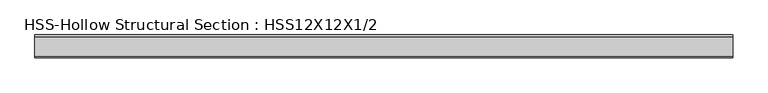
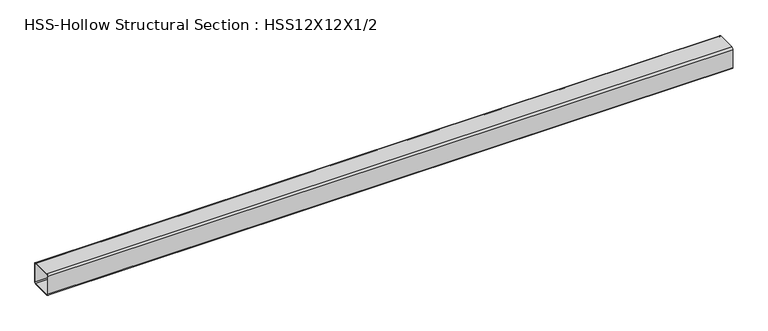
"""IFC4 building model written with IfcOpenShell, lengths in millimetres: beam geometry, HSS-Hollow Structural Section : HSS12X12X1/2."""

import ifcopenshell
import ifcopenshell.guid

model = None  # the IFC model being written
_history = None  # IfcOwnerHistory: only IFC2X3 demands one
_inside = {}  # id of a spatial element -> (the spatial element, [elements in it])
_under = {}  # id of a project, library or spatial element -> (it, [spatial elements below it])
_declared = {}  # id of a project -> (the project, [libraries it declares])
_typed = {}  # id of a type object -> (the type object, [elements of that type])
_made_of = {}  # id of a material, layer set ... -> (it, [elements and type objects made of it])


def new_model(schema):
    """Start an empty IFC model of exactly this schema.

    Asked for "IFC4X3", IfcOpenShell would pick the latest addendum, in which some entities
    have other attributes; the version numbers below select the first issue.
    IFC2X3 requires an IfcOwnerHistory on every rooted entity: one is made here for all.
    """
    global model, _history
    if schema == "IFC4X3":
        model = ifcopenshell.file(schema_version=(4, 3, 0, 0))
    else:
        model = ifcopenshell.file(schema=schema)
    _inside.clear()
    _under.clear()
    _declared.clear()
    _typed.clear()
    _made_of.clear()
    _history = None
    if model.schema == "IFC2X3":
        org = make("IfcOrganization", Name="unknown")
        user = make(
            "IfcPersonAndOrganization",
            ThePerson=make("IfcPerson", FamilyName="unknown"),
            TheOrganization=org,
        )
        app = make(
            "IfcApplication",
            ApplicationDeveloper=org,
            Version="unknown",
            ApplicationFullName="unknown",
            ApplicationIdentifier="unknown",
        )
        _history = make(
            "IfcOwnerHistory",
            OwningUser=user,
            OwningApplication=app,
            ChangeAction="ADDED",
            CreationDate=0,
        )
    return model


def make(cls, **values):
    """One entity of the class cls with the attributes given. An attribute that is None is left unset."""
    return model.create_entity(
        cls, **{name: value for name, value in values.items() if value is not None}
    )


def rooted(cls, **values):
    """An entity with a GlobalId (a new one), such as an element, a storey or a relation."""
    return make(cls, GlobalId=ifcopenshell.guid.new(), OwnerHistory=_history, **values)


def si_unit(unit_type, name, prefix=None):
    """IfcSIUnit, for example si_unit("LENGTHUNIT", "METRE", prefix="MILLI")."""
    return make("IfcSIUnit", UnitType=unit_type, Prefix=prefix, Name=name)


def assignment(units):
    """IfcUnitAssignment: the units of a project."""
    return None if units is None else make("IfcUnitAssignment", Units=units)


def point(xyz):
    """IfcCartesianPoint."""
    return None if xyz is None else make("IfcCartesianPoint", Coordinates=xyz)


def direction(xyz):
    """IfcDirection."""
    return None if xyz is None else make("IfcDirection", DirectionRatios=xyz)


def frame(location, z_axis=None, x_axis=None):
    """IfcAxis2Placement3D, a coordinate frame: its origin and axes. An axis left out is left unset."""
    return make(
        "IfcAxis2Placement3D",
        Location=point(location),
        Axis=direction(z_axis),
        RefDirection=direction(x_axis),
    )


def frame_2d(location, x_axis=None):
    """IfcAxis2Placement2D, a coordinate frame in the plane: its origin and x axis."""
    return make(
        "IfcAxis2Placement2D", Location=point(location), RefDirection=direction(x_axis)
    )


def origin():
    """The frame at (0, 0, 0) with its axes left unset."""
    return frame((0.0, 0.0, 0.0))


def place(relative_to, where):
    """IfcLocalPlacement: puts the frame where relative to a parent placement (None: the world)."""
    return make(
        "IfcLocalPlacement", PlacementRelTo=relative_to, RelativePlacement=where
    )


def context(
    kind, dimensions, precision=None, world=None, true_north=None, identifier=None
):
    """IfcGeometricRepresentationContext, for example the 3D "Model" context."""
    return make(
        "IfcGeometricRepresentationContext",
        ContextIdentifier=identifier,
        ContextType=kind,
        CoordinateSpaceDimension=dimensions,
        Precision=precision,
        WorldCoordinateSystem=world,
        TrueNorth=true_north,
    )


def project(units=None, contexts=None):
    """IfcProject with its units and contexts."""
    return rooted(
        "IfcProject",
        Name="project",
        RepresentationContexts=contexts,
        UnitsInContext=assignment(units),
    )


def spatial(cls, under=None, at=None, **own):
    """A site, building, storey or space (cls), placed at a placement, below another one or the project."""
    s = rooted(cls, ObjectPlacement=at, **own)
    if under is not None:
        _under.setdefault(under.id(), (under, []))[1].append(s)
    return s


def polyline(points):
    """IfcPolyline through the points."""
    return make("IfcPolyline", Points=[point(p) for p in points])


def circle_curve(where, radius):
    """IfcCircle in the frame where."""
    return make("IfcCircle", Position=where, Radius=radius)


def trimmed(basis, trim1, trim2, sense, master):
    """IfcTrimmedCurve: the piece of a basis curve between two trims."""
    return make(
        "IfcTrimmedCurve",
        BasisCurve=basis,
        Trim1=trim1,
        Trim2=trim2,
        SenseAgreement=sense,
        MasterRepresentation=master,
    )


def segment(curve, same_sense, transition):
    """IfcCompositeCurveSegment."""
    return make(
        "IfcCompositeCurveSegment",
        Transition=transition,
        SameSense=same_sense,
        ParentCurve=curve,
    )


def composite_curve(segments, self_intersect=None):
    """IfcCompositeCurve: segments joined end to end."""
    return make("IfcCompositeCurve", Segments=segments, SelfIntersect=self_intersect)


def outline(outer, holes=None, kind="AREA"):
    """IfcArbitraryClosedProfileDef: a profile drawn as a closed curve; with holes, ...WithVoids."""
    if holes is None:
        return make("IfcArbitraryClosedProfileDef", ProfileType=kind, OuterCurve=outer)
    return make(
        "IfcArbitraryProfileDefWithVoids",
        ProfileType=kind,
        OuterCurve=outer,
        InnerCurves=holes,
    )


def extrude(swept, where, along, depth):
    """IfcExtrudedAreaSolid: the profile swept, set in the frame where, extruded along a direction by depth."""
    return make(
        "IfcExtrudedAreaSolid",
        SweptArea=swept,
        Position=where,
        ExtrudedDirection=direction(along),
        Depth=depth,
    )


def shape(context_of_items, identifier, shape_type, items):
    """IfcShapeRepresentation: the items that make up one representation, for example the "Body"."""
    return make(
        "IfcShapeRepresentation",
        ContextOfItems=context_of_items,
        RepresentationIdentifier=identifier,
        RepresentationType=shape_type,
        Items=items,
    )


def source(mapping_origin, context_of_items, identifier, shape_type, items):
    """IfcRepresentationMap: a shape defined once, which mapped items show again and again."""
    return make(
        "IfcRepresentationMap",
        MappingOrigin=mapping_origin,
        MappedRepresentation=shape(context_of_items, identifier, shape_type, items),
    )


def transform(
    local_origin,
    x_axis=None,
    y_axis=None,
    z_axis=None,
    scale=None,
    scale2=None,
    scale3=None,
    uniform=True,
):
    """IfcCartesianTransformationOperator3D, or its non-uniform kind. x_axis, y_axis, z_axis: its Axis1, 2, 3."""
    if uniform:
        return make(
            "IfcCartesianTransformationOperator3D",
            Axis1=direction(x_axis),
            Axis2=direction(y_axis),
            LocalOrigin=point(local_origin),
            Scale=scale,
            Axis3=direction(z_axis),
        )
    return make(
        "IfcCartesianTransformationOperator3DnonUniform",
        Axis1=direction(x_axis),
        Axis2=direction(y_axis),
        LocalOrigin=point(local_origin),
        Scale=scale,
        Axis3=direction(z_axis),
        Scale2=scale2,
        Scale3=scale3,
    )


def mapped(mapping_source, mapping_target):
    """IfcMappedItem: shows the shape of a source again, moved by a transform."""
    return make(
        "IfcMappedItem", MappingSource=mapping_source, MappingTarget=mapping_target
    )


def made_of(thing, what):
    """Note that an element or type object is made of a material, layer set ...; save() writes the relation."""
    if what is not None:
        _made_of.setdefault(what.id(), (what, []))[1].append(thing)
    return thing


def element(
    cls,
    number,
    at=None,
    inside=None,
    cuts=None,
    type_object=None,
    material=None,
    context=None,
    identifier="Body",
    shape_type=None,
    held_by="IfcProductDefinitionShape",
    body=None,
    shapes=None,
    **own,
):
    """One element of the class cls, such as IfcWall. Its Tag is "e" and its number.

    at: its placement. inside: the storey or other place that contains it. cuts: it is an
    opening in that element (IfcRelVoidsElement). A single representation is given by context,
    identifier, shape_type and body (its items); several are given by shapes. held_by: the class
    of the entity that holds the representations. save() writes the other relations.
    """
    e = rooted(cls, Tag="e%d" % number, ObjectPlacement=at, **own)
    if body is not None:
        shapes = [shape(context, identifier, shape_type, body)]
    if shapes is not None:
        e.Representation = make(held_by, Representations=shapes)
    if inside is not None:
        _inside.setdefault(inside.id(), (inside, []))[1].append(e)
    if cuts is not None:
        rooted(
            "IfcRelVoidsElement", RelatingBuildingElement=cuts, RelatedOpeningElement=e
        )
    if type_object is not None:
        _typed.setdefault(type_object.id(), (type_object, []))[1].append(e)
    return made_of(e, material)


def aggregate(whole, parts):
    """IfcRelAggregates: a whole, such as a stair, and the parts it consists of."""
    return rooted("IfcRelAggregates", RelatingObject=whole, RelatedObjects=parts)


def save(model, path):
    """Write the relations noted so far, then the file.

    IfcRelAggregates (storeys below a building ...), IfcRelContainedInSpatialStructure (elements
    in a storey), IfcRelDefinesByType, IfcRelAssociatesMaterial and IfcRelDeclares: one each for
    every whole, place, type object, material and project.
    """
    for whole, parts in _under.values():
        aggregate(whole, parts)
    for where, things in _inside.values():
        rooted(
            "IfcRelContainedInSpatialStructure",
            RelatedElements=things,
            RelatingStructure=where,
        )
    for kind, things in _typed.values():
        rooted("IfcRelDefinesByType", RelatedObjects=things, RelatingType=kind)
    for what, things in _made_of.values():
        rooted("IfcRelAssociatesMaterial", RelatedObjects=things, RelatingMaterial=what)
    for by, libraries in _declared.values():
        rooted("IfcRelDeclares", RelatingContext=by, RelatedDefinitions=libraries)
    model.write(path)


def hss_hollow_structural_section_hss12x12x1_2_15489e63(model_context):
    return source(origin(), model_context, "Body", "SweptSolid", [
        extrude(outline(composite_curve([segment(polyline([(152.4, 128.778), (152.4, -128.778)]), True, "CONTINUOUS"), segment(trimmed(circle_curve(frame_2d((128.778, -128.778)), 23.622), [point((152.4, -128.778))], [point((128.778, -152.4))], False, "CARTESIAN"), True, "CONTINUOUS"), segment(polyline([(128.778, -152.4), (-128.778, -152.4)]), True, "CONTINUOUS"), segment(trimmed(circle_curve(frame_2d((-128.778, -128.778)), 23.622), [point((-128.778, -152.4))], [point((-152.4, -128.778))], False, "CARTESIAN"), True, "CONTINUOUS"), segment(polyline([(-152.4, -128.778), (-152.4, 128.778)]), True, "CONTINUOUS"), segment(trimmed(circle_curve(frame_2d((-128.778, 128.778)), 23.622), [point((-152.4, 128.778))], [point((-128.778, 152.4))], False, "CARTESIAN"), True, "CONTINUOUS"), segment(polyline([(-128.778, 152.4), (128.778, 152.4)]), True, "CONTINUOUS"), segment(trimmed(circle_curve(frame_2d((128.778, 128.778)), 23.622), [point((128.778, 152.4))], [point((152.4, 128.778))], False, "CARTESIAN"), True, "CONTINUOUS")], self_intersect=False), holes=[composite_curve([segment(trimmed(circle_curve(frame_2d((-128.778, 128.778)), 11.811), [point((-128.778, 140.589))], [point((-140.589, 128.778))], True, "CARTESIAN"), True, "CONTINUOUS"), segment(polyline([(-140.589, 128.778), (-140.589, -128.778)]), True, "CONTINUOUS"), segment(trimmed(circle_curve(frame_2d((-128.778, -128.778)), 11.811), [point((-140.589, -128.778))], [point((-128.778, -140.589))], True, "CARTESIAN"), True, "CONTINUOUS"), segment(polyline([(-128.778, -140.589), (128.778, -140.589)]), True, "CONTINUOUS"), segment(trimmed(circle_curve(frame_2d((128.778, -128.778)), 11.811), [point((128.778, -140.589))], [point((140.589, -128.778))], True, "CARTESIAN"), True, "CONTINUOUS"), segment(polyline([(140.589, -128.778), (140.589, 128.778)]), True, "CONTINUOUS"), segment(trimmed(circle_curve(frame_2d((128.778, 128.778)), 11.811), [point((140.589, 128.778))], [point((128.778, 140.589))], True, "CARTESIAN"), True, "CONTINUOUS"), segment(polyline([(128.778, 140.589), (-128.778, 140.589)]), True, "CONTINUOUS")], self_intersect=False)]), frame((-4705.6506621, 0.0, 0.0), z_axis=(1.0, 0.0, 0.0), x_axis=(0.0, 1.0, 0.0)), (0.0, 0.0, 1.0), 9257.1223245),
    ])


if __name__ == "__main__":
    model = new_model("IFC4")
    model_context = context("Model", 3, world=origin())
    ifc_project = project(units=[si_unit("LENGTHUNIT", "METRE", prefix="MILLI")], contexts=[model_context])
    site = spatial("IfcSite", under=ifc_project)
    building = spatial("IfcBuilding", under=site)
    placement = place(None, origin())
    hss_hollow_structural_section_hss12x12x1_2_shape = hss_hollow_structural_section_hss12x12x1_2_15489e63(model_context)
    element("IfcBeam", 1, ObjectType="HSS-Hollow Structural Section : HSS12X12X1/2", at=placement, inside=building, context=model_context, shape_type="MappedRepresentation", body=[
        mapped(hss_hollow_structural_section_hss12x12x1_2_shape, transform((0.0, 0.0, 0.0), x_axis=(1.0, 0.0, 0.0), y_axis=(0.0, 1.0, 0.0), z_axis=(0.0, 0.0, 1.0))),
    ])
    save(model, "model.ifc")

# Revit data of these elements
# Type "HSS-Hollow Structural Section : HSS12X12X1/2"
#   Assembly Code = "B10"
#   Shape = "Square"
#   W = 75.9
#   Ht = 304.8 mm
#   Length [instance default] = 1524 mm
#   b = 304.8 mm
#   kr = 23.622 mm
#   t = 11.811 mm
#   A = 0.0134838 m²
#   Structural Material [instance default] = Steel ASTM A500, Grade B, Rectangular and Square
# Element 1 (IfcBeam, "HSS-Hollow Structural Section : HSS12X12X1/2")
#   Structural Material = Aluminum 7175 T73 0 Hot Formed
#   Materials on its faces: "Aluminum 7175 T73 0 Hot Formed"
# Materials
#   "Steel ASTM A500, Grade B, Rectangular and Square": class "Metal", colour RGB 199 199 199, transparency 0, Description = "Carbon steel", Cost = 0
#   "Aluminum 7175 T73 0 Hot Formed": class "Metal", colour RGB 120 120 120, transparency 0, Description = "Physical material.", Cost = 0
